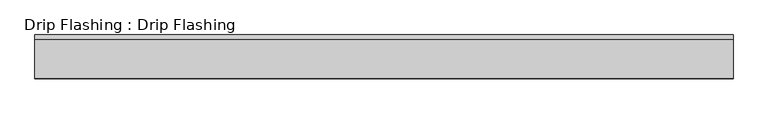
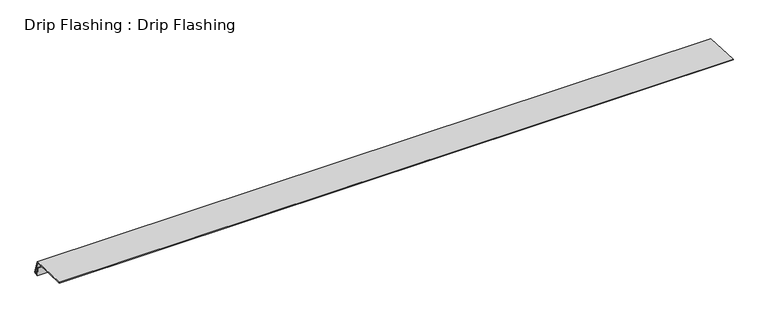
"""IFC4 building model written with IfcOpenShell, lengths in millimetres: proxy geometry, Drip Flashing : Drip Flashing."""

from ifc_helpers import new_model, si_unit, frame, origin, place, context, project, spatial, polyline, outline, extrude, source, transform, mapped, element, save


def drip_flashing_drip_flashing_05063a31(model_context):
    return source(origin(), model_context, "Body", "SweptSolid", [
        extrude(outline(polyline([(9772.4316207, 37600.241418), (9660.1127629, 37604.8160522), (9660.1989012, 37606.9309658), (9774.0264732, 37602.2948832), (9786.1199219, 37561.887738), (9774.040701, 37558.2725497), (9771.4197382, 37583.2093446), (9773.5082342, 37583.4288544), (9775.8645053, 37561.0104321), (9783.490007, 37563.2926674), (9772.4316207, 37600.241418)])), frame((-9232.0719278, 0.0, 0.0), z_axis=(1.0, 0.0, 0.0), x_axis=(0.0, 1.0, 0.0)), (0.0, 0.0, 1.0), 1999.85),
    ])


if __name__ == "__main__":
    model = new_model("IFC4")
    model_context = context("Model", 3, world=origin())
    ifc_project = project(units=[si_unit("LENGTHUNIT", "METRE", prefix="MILLI")], contexts=[model_context])
    site = spatial("IfcSite", under=ifc_project)
    building = spatial("IfcBuilding", under=site)
    placement = place(None, origin())
    drip_flashing_drip_flashing_shape = drip_flashing_drip_flashing_05063a31(model_context)
    element("IfcBuildingElementProxy", 1, Name="Drip Flashing : Drip Flashing", ObjectType="Drip Flashing : Drip Flashing", at=placement, inside=building, context=model_context, shape_type="MappedRepresentation", body=[
        mapped(drip_flashing_drip_flashing_shape, transform((0.0, 0.0, 0.0), x_axis=(1.0, 0.0, 0.0), y_axis=(0.0, 1.0, 0.0), z_axis=(0.0, 0.0, 1.0))),
    ])
    save(model, "model.ifc")

# Revit data of these elements
# Type "Drip Flashing : Drip Flashing"
#   NameOverride = "Drip Flashing"
# Element 1 (IfcBuildingElementProxy, "Drip Flashing : Drip Flashing")
#   Materials on its faces: "DRIP FLASHING"
# Materials
#   "DRIP FLASHING": class "Unassigned", colour RGB 134 230 106, transparency 0, Cost = 0
